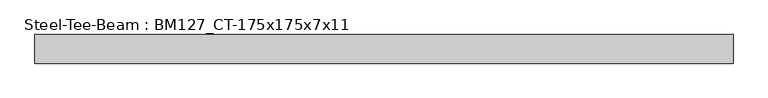
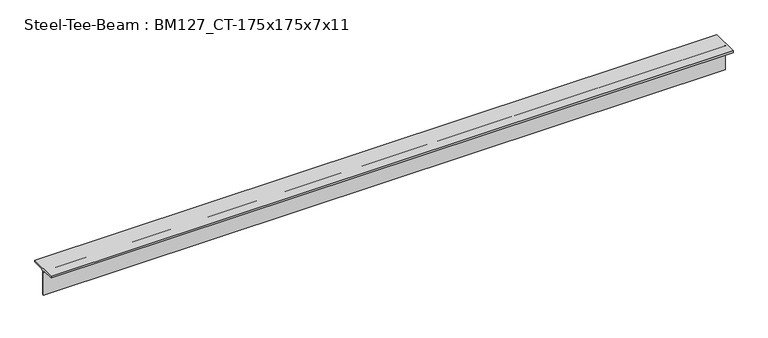
"""IFC4 building model written with IfcOpenShell, lengths in millimetres: beam geometry, Steel-Tee-Beam : BM127_CT-175x175x7x11."""

import ifcopenshell
import ifcopenshell.guid

model = None  # the IFC model being written
_history = None  # IfcOwnerHistory: only IFC2X3 demands one
_inside = {}  # id of a spatial element -> (the spatial element, [elements in it])
_under = {}  # id of a project, library or spatial element -> (it, [spatial elements below it])
_declared = {}  # id of a project -> (the project, [libraries it declares])
_typed = {}  # id of a type object -> (the type object, [elements of that type])
_made_of = {}  # id of a material, layer set ... -> (it, [elements and type objects made of it])


def new_model(schema):
    """Start an empty IFC model of exactly this schema.

    Asked for "IFC4X3", IfcOpenShell would pick the latest addendum, in which some entities
    have other attributes; the version numbers below select the first issue.
    IFC2X3 requires an IfcOwnerHistory on every rooted entity: one is made here for all.
    """
    global model, _history
    if schema == "IFC4X3":
        model = ifcopenshell.file(schema_version=(4, 3, 0, 0))
    else:
        model = ifcopenshell.file(schema=schema)
    _inside.clear()
    _under.clear()
    _declared.clear()
    _typed.clear()
    _made_of.clear()
    _history = None
    if model.schema == "IFC2X3":
        org = make("IfcOrganization", Name="unknown")
        user = make(
            "IfcPersonAndOrganization",
            ThePerson=make("IfcPerson", FamilyName="unknown"),
            TheOrganization=org,
        )
        app = make(
            "IfcApplication",
            ApplicationDeveloper=org,
            Version="unknown",
            ApplicationFullName="unknown",
            ApplicationIdentifier="unknown",
        )
        _history = make(
            "IfcOwnerHistory",
            OwningUser=user,
            OwningApplication=app,
            ChangeAction="ADDED",
            CreationDate=0,
        )
    return model


def make(cls, **values):
    """One entity of the class cls with the attributes given. An attribute that is None is left unset."""
    return model.create_entity(
        cls, **{name: value for name, value in values.items() if value is not None}
    )


def rooted(cls, **values):
    """An entity with a GlobalId (a new one), such as an element, a storey or a relation."""
    return make(cls, GlobalId=ifcopenshell.guid.new(), OwnerHistory=_history, **values)


def si_unit(unit_type, name, prefix=None):
    """IfcSIUnit, for example si_unit("LENGTHUNIT", "METRE", prefix="MILLI")."""
    return make("IfcSIUnit", UnitType=unit_type, Prefix=prefix, Name=name)


def assignment(units):
    """IfcUnitAssignment: the units of a project."""
    return None if units is None else make("IfcUnitAssignment", Units=units)


def point(xyz):
    """IfcCartesianPoint."""
    return None if xyz is None else make("IfcCartesianPoint", Coordinates=xyz)


def direction(xyz):
    """IfcDirection."""
    return None if xyz is None else make("IfcDirection", DirectionRatios=xyz)


def frame(location, z_axis=None, x_axis=None):
    """IfcAxis2Placement3D, a coordinate frame: its origin and axes. An axis left out is left unset."""
    return make(
        "IfcAxis2Placement3D",
        Location=point(location),
        Axis=direction(z_axis),
        RefDirection=direction(x_axis),
    )


def frame_2d(location, x_axis=None):
    """IfcAxis2Placement2D, a coordinate frame in the plane: its origin and x axis."""
    return make(
        "IfcAxis2Placement2D", Location=point(location), RefDirection=direction(x_axis)
    )


def origin():
    """The frame at (0, 0, 0) with its axes left unset."""
    return frame((0.0, 0.0, 0.0))


def place(relative_to, where):
    """IfcLocalPlacement: puts the frame where relative to a parent placement (None: the world)."""
    return make(
        "IfcLocalPlacement", PlacementRelTo=relative_to, RelativePlacement=where
    )


def context(
    kind, dimensions, precision=None, world=None, true_north=None, identifier=None
):
    """IfcGeometricRepresentationContext, for example the 3D "Model" context."""
    return make(
        "IfcGeometricRepresentationContext",
        ContextIdentifier=identifier,
        ContextType=kind,
        CoordinateSpaceDimension=dimensions,
        Precision=precision,
        WorldCoordinateSystem=world,
        TrueNorth=true_north,
    )


def project(units=None, contexts=None):
    """IfcProject with its units and contexts."""
    return rooted(
        "IfcProject",
        Name="project",
        RepresentationContexts=contexts,
        UnitsInContext=assignment(units),
    )


def spatial(cls, under=None, at=None, **own):
    """A site, building, storey or space (cls), placed at a placement, below another one or the project."""
    s = rooted(cls, ObjectPlacement=at, **own)
    if under is not None:
        _under.setdefault(under.id(), (under, []))[1].append(s)
    return s


def polyline(points):
    """IfcPolyline through the points."""
    return make("IfcPolyline", Points=[point(p) for p in points])


def circle_curve(where, radius):
    """IfcCircle in the frame where."""
    return make("IfcCircle", Position=where, Radius=radius)


def trimmed(basis, trim1, trim2, sense, master):
    """IfcTrimmedCurve: the piece of a basis curve between two trims."""
    return make(
        "IfcTrimmedCurve",
        BasisCurve=basis,
        Trim1=trim1,
        Trim2=trim2,
        SenseAgreement=sense,
        MasterRepresentation=master,
    )


def segment(curve, same_sense, transition):
    """IfcCompositeCurveSegment."""
    return make(
        "IfcCompositeCurveSegment",
        Transition=transition,
        SameSense=same_sense,
        ParentCurve=curve,
    )


def composite_curve(segments, self_intersect=None):
    """IfcCompositeCurve: segments joined end to end."""
    return make("IfcCompositeCurve", Segments=segments, SelfIntersect=self_intersect)


def outline(outer, holes=None, kind="AREA"):
    """IfcArbitraryClosedProfileDef: a profile drawn as a closed curve; with holes, ...WithVoids."""
    if holes is None:
        return make("IfcArbitraryClosedProfileDef", ProfileType=kind, OuterCurve=outer)
    return make(
        "IfcArbitraryProfileDefWithVoids",
        ProfileType=kind,
        OuterCurve=outer,
        InnerCurves=holes,
    )


def extrude(swept, where, along, depth):
    """IfcExtrudedAreaSolid: the profile swept, set in the frame where, extruded along a direction by depth."""
    return make(
        "IfcExtrudedAreaSolid",
        SweptArea=swept,
        Position=where,
        ExtrudedDirection=direction(along),
        Depth=depth,
    )


def shape(context_of_items, identifier, shape_type, items):
    """IfcShapeRepresentation: the items that make up one representation, for example the "Body"."""
    return make(
        "IfcShapeRepresentation",
        ContextOfItems=context_of_items,
        RepresentationIdentifier=identifier,
        RepresentationType=shape_type,
        Items=items,
    )


def source(mapping_origin, context_of_items, identifier, shape_type, items):
    """IfcRepresentationMap: a shape defined once, which mapped items show again and again."""
    return make(
        "IfcRepresentationMap",
        MappingOrigin=mapping_origin,
        MappedRepresentation=shape(context_of_items, identifier, shape_type, items),
    )


def transform(
    local_origin,
    x_axis=None,
    y_axis=None,
    z_axis=None,
    scale=None,
    scale2=None,
    scale3=None,
    uniform=True,
):
    """IfcCartesianTransformationOperator3D, or its non-uniform kind. x_axis, y_axis, z_axis: its Axis1, 2, 3."""
    if uniform:
        return make(
            "IfcCartesianTransformationOperator3D",
            Axis1=direction(x_axis),
            Axis2=direction(y_axis),
            LocalOrigin=point(local_origin),
            Scale=scale,
            Axis3=direction(z_axis),
        )
    return make(
        "IfcCartesianTransformationOperator3DnonUniform",
        Axis1=direction(x_axis),
        Axis2=direction(y_axis),
        LocalOrigin=point(local_origin),
        Scale=scale,
        Axis3=direction(z_axis),
        Scale2=scale2,
        Scale3=scale3,
    )


def mapped(mapping_source, mapping_target):
    """IfcMappedItem: shows the shape of a source again, moved by a transform."""
    return make(
        "IfcMappedItem", MappingSource=mapping_source, MappingTarget=mapping_target
    )


def made_of(thing, what):
    """Note that an element or type object is made of a material, layer set ...; save() writes the relation."""
    if what is not None:
        _made_of.setdefault(what.id(), (what, []))[1].append(thing)
    return thing


def element(
    cls,
    number,
    at=None,
    inside=None,
    cuts=None,
    type_object=None,
    material=None,
    context=None,
    identifier="Body",
    shape_type=None,
    held_by="IfcProductDefinitionShape",
    body=None,
    shapes=None,
    **own,
):
    """One element of the class cls, such as IfcWall. Its Tag is "e" and its number.

    at: its placement. inside: the storey or other place that contains it. cuts: it is an
    opening in that element (IfcRelVoidsElement). A single representation is given by context,
    identifier, shape_type and body (its items); several are given by shapes. held_by: the class
    of the entity that holds the representations. save() writes the other relations.
    """
    e = rooted(cls, Tag="e%d" % number, ObjectPlacement=at, **own)
    if body is not None:
        shapes = [shape(context, identifier, shape_type, body)]
    if shapes is not None:
        e.Representation = make(held_by, Representations=shapes)
    if inside is not None:
        _inside.setdefault(inside.id(), (inside, []))[1].append(e)
    if cuts is not None:
        rooted(
            "IfcRelVoidsElement", RelatingBuildingElement=cuts, RelatedOpeningElement=e
        )
    if type_object is not None:
        _typed.setdefault(type_object.id(), (type_object, []))[1].append(e)
    return made_of(e, material)


def aggregate(whole, parts):
    """IfcRelAggregates: a whole, such as a stair, and the parts it consists of."""
    return rooted("IfcRelAggregates", RelatingObject=whole, RelatedObjects=parts)


def save(model, path):
    """Write the relations noted so far, then the file.

    IfcRelAggregates (storeys below a building ...), IfcRelContainedInSpatialStructure (elements
    in a storey), IfcRelDefinesByType, IfcRelAssociatesMaterial and IfcRelDeclares: one each for
    every whole, place, type object, material and project.
    """
    for whole, parts in _under.values():
        aggregate(whole, parts)
    for where, things in _inside.values():
        rooted(
            "IfcRelContainedInSpatialStructure",
            RelatedElements=things,
            RelatingStructure=where,
        )
    for kind, things in _typed.values():
        rooted("IfcRelDefinesByType", RelatedObjects=things, RelatingType=kind)
    for what, things in _made_of.values():
        rooted("IfcRelAssociatesMaterial", RelatedObjects=things, RelatingMaterial=what)
    for by, libraries in _declared.values():
        rooted("IfcRelDeclares", RelatingContext=by, RelatedDefinitions=libraries)
    model.write(path)


def steel_tee_beam_bm127_ct_175x175x7x11_58f75cbf(model_context):
    return source(origin(), model_context, "Body", "SweptSolid", [
        extrude(outline(composite_curve([segment(polyline([(-87.5, 87.5), (87.5, 87.5), (87.5, 76.5), (17.5, 76.5)]), True, "CONTINUOUS"), segment(trimmed(circle_curve(frame_2d((17.5, 62.5)), 14.0), [point((17.5, 76.5))], [point((3.5, 62.5))], True, "CARTESIAN"), True, "CONTINUOUS"), segment(polyline([(3.5, 62.5), (3.5, -87.5), (-3.5, -87.5), (-3.5, 62.5)]), True, "CONTINUOUS"), segment(trimmed(circle_curve(frame_2d((-17.5, 62.5)), 14.0), [point((-3.5, 62.5))], [point((-17.5, 76.5))], True, "CARTESIAN"), True, "CONTINUOUS"), segment(polyline([(-17.5, 76.5), (-87.5, 76.5), (-87.5, 87.5)]), True, "CONTINUOUS")], self_intersect=False)), frame((-2077.083277, 0.0, 0.0), z_axis=(1.0, 0.0, 0.0), x_axis=(0.0, 1.0, 0.0)), (0.0, 0.0, 1.0), 4261.3199196),
    ])


if __name__ == "__main__":
    model = new_model("IFC4")
    model_context = context("Model", 3, world=origin())
    ifc_project = project(units=[si_unit("LENGTHUNIT", "METRE", prefix="MILLI")], contexts=[model_context])
    site = spatial("IfcSite", under=ifc_project)
    building = spatial("IfcBuilding", under=site)
    placement = place(None, origin())
    steel_tee_beam_bm127_ct_175x175x7x11_shape = steel_tee_beam_bm127_ct_175x175x7x11_58f75cbf(model_context)
    element("IfcBeam", 1, ObjectType="Steel-Tee-Beam : BM127_CT-175x175x7x11", at=placement, inside=building, context=model_context, shape_type="MappedRepresentation", body=[
        mapped(steel_tee_beam_bm127_ct_175x175x7x11_shape, transform((0.0, 0.0, 0.0), x_axis=(1.0, 0.0, 0.0), y_axis=(0.0, 1.0, 0.0), z_axis=(0.0, 0.0, 1.0))),
    ])
    save(model, "model.ifc")

# Revit data of these elements
# Type "Steel-Tee-Beam : BM127_CT-175x175x7x11"
#   Surface Area = 0.00 m²/m
#   Section Area = 31.57 cm²
#   Mass per Unit Length = 24.80 kg/m
#   Length [instance default] = 1524 mm
#   bf = 175 mm
#   d = 175 mm
#   k = 25 mm
#   kr = 14 mm
#   tf = 11 mm
#   tw = 7 mm
#   hec_material4 [instance default] = none
#   hec_material3 [instance default] = none
#   hec_material2 [instance default] = none
#   hec_material1 [instance default] = none
#   Structural Material [instance default] = Steel, 45-345
#   Assembly Code = ""
# Element 1 (IfcBeam, "Steel-Tee-Beam : BM127_CT-175x175x7x11")
#   hec_material3 = F01AC000-00002_Building/Shelter Fire Proofing Work_Intumescent Coating Type_1 hr. rating (UL 1709))
#   hec_material2 = S01AA010-00002_Main Steel Structure Fabrication Work_Shelter/Building_Steel Painting/Coating_for Fireproofed Steel Surface, Surface Preparation & Primer Coat
#   hec_material1 = S03AA029-00001_Main Steel Structure Erection Work_Shelter/Building_Light Steel
#   Structural Material = S01AA003-00001_Main Steel Structure Fabrication Work_Shelter/Building_Light Steel - Standard
#   Materials on its faces: "S01AA003-00001_Main Steel Structure Fabrication Work_Shelter/Building_Light Steel - Standard"
# Materials
#   "Steel, 45-345": class "Metal", colour RGB 189 187 185, transparency 0, Description = "Steel 345 MPa", Cost = 0
#   "S01AA003-00001_Main Steel Structure Fabrication Work_Shelter/Building_Light Steel - Standard": class "Metal", colour RGB 120 120 120, transparency 0, Comments = "(30KG/M>Weight)", Description = "Structural steel 50ksi", W00) Work Master Code = "S01AA003-00001", W01) Work Master_Lv1 = "Main Steel Structure Fabrication Work", W02) Work Master_Lv2 = "Shelter/Building", W03) Work Master_Spec.1 = "Light Steel - Standard (30KG/M>Weight)", Cost = 0
#   "F01AC000-00002_Building/Shelter Fire Proofing Work_Intumescent Coating Type_1 hr. rating (UL 1709))": class "Metal", colour RGB 255 128 128, transparency 0, Description = "Paint finished steel", W00) Work Master Code = "F01AC000-00002", W01) Work Master_Lv1 = "Building/Shelter Fire Proofing Work", W02) Work Master_Lv2 = "Intumescent Coating Type", W03) Work Master_Spec.1 = "1 hr. rating (UL 1709)", Cost = 0
#   "S01AA010-00002_Main Steel Structure Fabrication Work_Shelter/Building_Steel Painting/Coating_for Fireproofed Steel Surface, Surface Preparation & Primer Coat": class "Metal", colour RGB 120 120 120, transparency 0, Description = "Paint finished steel", W00) Work Master Code = "SS01AA010-00002", W01) Work Master_Lv1 = "Main Steel Structure Fabrication Work", W02) Work Master_Lv2 = "Shelter/Building", W03) Work Master_Spec.1 = "Steel Painting/Coating", W04) Work Master_Spec.2 = "for Fireproofed Steel Surface, Surface Preparation & Primer Coat", Cost = 0
#   "S03AA029-00001_Main Steel Structure Erection Work_Shelter/Building_Light Steel": class "Metal", colour RGB 120 120 120, transparency 0, Comments = "(30KG/M>Weight)", Description = "Structural steel 50ksi", W00) Work Master Code = "S03AA029-00001", W01) Work Master_Lv1 = "Main Steel Structure Erection Work", W02) Work Master_Lv2 = "Shelter/Building", W03) Work Master_Spec.1 = "Light Steel (30KG/M>Weight)", Cost = 0
